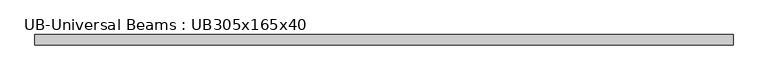
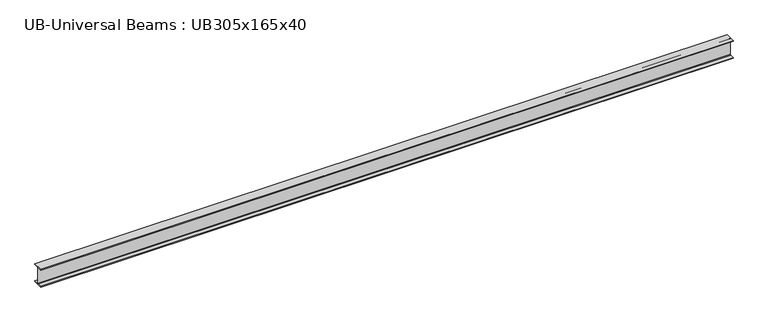
"""IFC4 building model written with IfcOpenShell, lengths in millimetres: member geometry, UB-Universal Beams : UB305x165x40."""

import ifcopenshell
import ifcopenshell.guid

model = None  # the IFC model being written
_history = None  # IfcOwnerHistory: only IFC2X3 demands one
_inside = {}  # id of a spatial element -> (the spatial element, [elements in it])
_under = {}  # id of a project, library or spatial element -> (it, [spatial elements below it])
_declared = {}  # id of a project -> (the project, [libraries it declares])
_typed = {}  # id of a type object -> (the type object, [elements of that type])
_made_of = {}  # id of a material, layer set ... -> (it, [elements and type objects made of it])


def new_model(schema):
    """Start an empty IFC model of exactly this schema.

    Asked for "IFC4X3", IfcOpenShell would pick the latest addendum, in which some entities
    have other attributes; the version numbers below select the first issue.
    IFC2X3 requires an IfcOwnerHistory on every rooted entity: one is made here for all.
    """
    global model, _history
    if schema == "IFC4X3":
        model = ifcopenshell.file(schema_version=(4, 3, 0, 0))
    else:
        model = ifcopenshell.file(schema=schema)
    _inside.clear()
    _under.clear()
    _declared.clear()
    _typed.clear()
    _made_of.clear()
    _history = None
    if model.schema == "IFC2X3":
        org = make("IfcOrganization", Name="unknown")
        user = make(
            "IfcPersonAndOrganization",
            ThePerson=make("IfcPerson", FamilyName="unknown"),
            TheOrganization=org,
        )
        app = make(
            "IfcApplication",
            ApplicationDeveloper=org,
            Version="unknown",
            ApplicationFullName="unknown",
            ApplicationIdentifier="unknown",
        )
        _history = make(
            "IfcOwnerHistory",
            OwningUser=user,
            OwningApplication=app,
            ChangeAction="ADDED",
            CreationDate=0,
        )
    return model


def make(cls, **values):
    """One entity of the class cls with the attributes given. An attribute that is None is left unset."""
    return model.create_entity(
        cls, **{name: value for name, value in values.items() if value is not None}
    )


def rooted(cls, **values):
    """An entity with a GlobalId (a new one), such as an element, a storey or a relation."""
    return make(cls, GlobalId=ifcopenshell.guid.new(), OwnerHistory=_history, **values)


def si_unit(unit_type, name, prefix=None):
    """IfcSIUnit, for example si_unit("LENGTHUNIT", "METRE", prefix="MILLI")."""
    return make("IfcSIUnit", UnitType=unit_type, Prefix=prefix, Name=name)


def assignment(units):
    """IfcUnitAssignment: the units of a project."""
    return None if units is None else make("IfcUnitAssignment", Units=units)


def point(xyz):
    """IfcCartesianPoint."""
    return None if xyz is None else make("IfcCartesianPoint", Coordinates=xyz)


def direction(xyz):
    """IfcDirection."""
    return None if xyz is None else make("IfcDirection", DirectionRatios=xyz)


def frame(location, z_axis=None, x_axis=None):
    """IfcAxis2Placement3D, a coordinate frame: its origin and axes. An axis left out is left unset."""
    return make(
        "IfcAxis2Placement3D",
        Location=point(location),
        Axis=direction(z_axis),
        RefDirection=direction(x_axis),
    )


def frame_2d(location, x_axis=None):
    """IfcAxis2Placement2D, a coordinate frame in the plane: its origin and x axis."""
    return make(
        "IfcAxis2Placement2D", Location=point(location), RefDirection=direction(x_axis)
    )


def origin():
    """The frame at (0, 0, 0) with its axes left unset."""
    return frame((0.0, 0.0, 0.0))


def place(relative_to, where):
    """IfcLocalPlacement: puts the frame where relative to a parent placement (None: the world)."""
    return make(
        "IfcLocalPlacement", PlacementRelTo=relative_to, RelativePlacement=where
    )


def context(
    kind, dimensions, precision=None, world=None, true_north=None, identifier=None
):
    """IfcGeometricRepresentationContext, for example the 3D "Model" context."""
    return make(
        "IfcGeometricRepresentationContext",
        ContextIdentifier=identifier,
        ContextType=kind,
        CoordinateSpaceDimension=dimensions,
        Precision=precision,
        WorldCoordinateSystem=world,
        TrueNorth=true_north,
    )


def project(units=None, contexts=None):
    """IfcProject with its units and contexts."""
    return rooted(
        "IfcProject",
        Name="project",
        RepresentationContexts=contexts,
        UnitsInContext=assignment(units),
    )


def spatial(cls, under=None, at=None, **own):
    """A site, building, storey or space (cls), placed at a placement, below another one or the project."""
    s = rooted(cls, ObjectPlacement=at, **own)
    if under is not None:
        _under.setdefault(under.id(), (under, []))[1].append(s)
    return s


def polyline(points):
    """IfcPolyline through the points."""
    return make("IfcPolyline", Points=[point(p) for p in points])


def circle_curve(where, radius):
    """IfcCircle in the frame where."""
    return make("IfcCircle", Position=where, Radius=radius)


def trimmed(basis, trim1, trim2, sense, master):
    """IfcTrimmedCurve: the piece of a basis curve between two trims."""
    return make(
        "IfcTrimmedCurve",
        BasisCurve=basis,
        Trim1=trim1,
        Trim2=trim2,
        SenseAgreement=sense,
        MasterRepresentation=master,
    )


def segment(curve, same_sense, transition):
    """IfcCompositeCurveSegment."""
    return make(
        "IfcCompositeCurveSegment",
        Transition=transition,
        SameSense=same_sense,
        ParentCurve=curve,
    )


def composite_curve(segments, self_intersect=None):
    """IfcCompositeCurve: segments joined end to end."""
    return make("IfcCompositeCurve", Segments=segments, SelfIntersect=self_intersect)


def outline(outer, holes=None, kind="AREA"):
    """IfcArbitraryClosedProfileDef: a profile drawn as a closed curve; with holes, ...WithVoids."""
    if holes is None:
        return make("IfcArbitraryClosedProfileDef", ProfileType=kind, OuterCurve=outer)
    return make(
        "IfcArbitraryProfileDefWithVoids",
        ProfileType=kind,
        OuterCurve=outer,
        InnerCurves=holes,
    )


def extrude(swept, where, along, depth):
    """IfcExtrudedAreaSolid: the profile swept, set in the frame where, extruded along a direction by depth."""
    return make(
        "IfcExtrudedAreaSolid",
        SweptArea=swept,
        Position=where,
        ExtrudedDirection=direction(along),
        Depth=depth,
    )


def shape(context_of_items, identifier, shape_type, items):
    """IfcShapeRepresentation: the items that make up one representation, for example the "Body"."""
    return make(
        "IfcShapeRepresentation",
        ContextOfItems=context_of_items,
        RepresentationIdentifier=identifier,
        RepresentationType=shape_type,
        Items=items,
    )


def source(mapping_origin, context_of_items, identifier, shape_type, items):
    """IfcRepresentationMap: a shape defined once, which mapped items show again and again."""
    return make(
        "IfcRepresentationMap",
        MappingOrigin=mapping_origin,
        MappedRepresentation=shape(context_of_items, identifier, shape_type, items),
    )


def transform(
    local_origin,
    x_axis=None,
    y_axis=None,
    z_axis=None,
    scale=None,
    scale2=None,
    scale3=None,
    uniform=True,
):
    """IfcCartesianTransformationOperator3D, or its non-uniform kind. x_axis, y_axis, z_axis: its Axis1, 2, 3."""
    if uniform:
        return make(
            "IfcCartesianTransformationOperator3D",
            Axis1=direction(x_axis),
            Axis2=direction(y_axis),
            LocalOrigin=point(local_origin),
            Scale=scale,
            Axis3=direction(z_axis),
        )
    return make(
        "IfcCartesianTransformationOperator3DnonUniform",
        Axis1=direction(x_axis),
        Axis2=direction(y_axis),
        LocalOrigin=point(local_origin),
        Scale=scale,
        Axis3=direction(z_axis),
        Scale2=scale2,
        Scale3=scale3,
    )


def mapped(mapping_source, mapping_target):
    """IfcMappedItem: shows the shape of a source again, moved by a transform."""
    return make(
        "IfcMappedItem", MappingSource=mapping_source, MappingTarget=mapping_target
    )


def made_of(thing, what):
    """Note that an element or type object is made of a material, layer set ...; save() writes the relation."""
    if what is not None:
        _made_of.setdefault(what.id(), (what, []))[1].append(thing)
    return thing


def element(
    cls,
    number,
    at=None,
    inside=None,
    cuts=None,
    type_object=None,
    material=None,
    context=None,
    identifier="Body",
    shape_type=None,
    held_by="IfcProductDefinitionShape",
    body=None,
    shapes=None,
    **own,
):
    """One element of the class cls, such as IfcWall. Its Tag is "e" and its number.

    at: its placement. inside: the storey or other place that contains it. cuts: it is an
    opening in that element (IfcRelVoidsElement). A single representation is given by context,
    identifier, shape_type and body (its items); several are given by shapes. held_by: the class
    of the entity that holds the representations. save() writes the other relations.
    """
    e = rooted(cls, Tag="e%d" % number, ObjectPlacement=at, **own)
    if body is not None:
        shapes = [shape(context, identifier, shape_type, body)]
    if shapes is not None:
        e.Representation = make(held_by, Representations=shapes)
    if inside is not None:
        _inside.setdefault(inside.id(), (inside, []))[1].append(e)
    if cuts is not None:
        rooted(
            "IfcRelVoidsElement", RelatingBuildingElement=cuts, RelatedOpeningElement=e
        )
    if type_object is not None:
        _typed.setdefault(type_object.id(), (type_object, []))[1].append(e)
    return made_of(e, material)


def aggregate(whole, parts):
    """IfcRelAggregates: a whole, such as a stair, and the parts it consists of."""
    return rooted("IfcRelAggregates", RelatingObject=whole, RelatedObjects=parts)


def save(model, path):
    """Write the relations noted so far, then the file.

    IfcRelAggregates (storeys below a building ...), IfcRelContainedInSpatialStructure (elements
    in a storey), IfcRelDefinesByType, IfcRelAssociatesMaterial and IfcRelDeclares: one each for
    every whole, place, type object, material and project.
    """
    for whole, parts in _under.values():
        aggregate(whole, parts)
    for where, things in _inside.values():
        rooted(
            "IfcRelContainedInSpatialStructure",
            RelatedElements=things,
            RelatingStructure=where,
        )
    for kind, things in _typed.values():
        rooted("IfcRelDefinesByType", RelatedObjects=things, RelatingType=kind)
    for what, things in _made_of.values():
        rooted("IfcRelAssociatesMaterial", RelatedObjects=things, RelatingMaterial=what)
    for by, libraries in _declared.values():
        rooted("IfcRelDeclares", RelatingContext=by, RelatedDefinitions=libraries)
    model.write(path)


def ub_universal_beams_ub305x165x40_967f8f3f(model_context):
    return source(origin(), model_context, "Body", "SweptSolid", [
        extrude(outline(composite_curve([segment(polyline([(82.5, -141.5), (82.5, -151.7), (-82.5, -151.7), (-82.5, -141.5), (-11.9, -141.5)]), True, "CONTINUOUS"), segment(trimmed(circle_curve(frame_2d((-11.9, -132.6)), 8.9), [point((-11.9, -141.5))], [point((-3.0, -132.6))], True, "CARTESIAN"), True, "CONTINUOUS"), segment(polyline([(-3.0, -132.6), (-3.0, 132.6)]), True, "CONTINUOUS"), segment(trimmed(circle_curve(frame_2d((-11.9, 132.6)), 8.9), [point((-3.0, 132.6))], [point((-11.9, 141.5))], True, "CARTESIAN"), True, "CONTINUOUS"), segment(polyline([(-11.9, 141.5), (-82.5, 141.5), (-82.5, 151.7), (82.5, 151.7), (82.5, 141.5), (11.9, 141.5)]), True, "CONTINUOUS"), segment(trimmed(circle_curve(frame_2d((11.9, 132.6)), 8.9), [point((11.9, 141.5))], [point((3.0, 132.6))], True, "CARTESIAN"), True, "CONTINUOUS"), segment(polyline([(3.0, 132.6), (3.0, -132.6)]), True, "CONTINUOUS"), segment(trimmed(circle_curve(frame_2d((11.9, -132.6)), 8.9), [point((3.0, -132.6))], [point((11.9, -141.5))], True, "CARTESIAN"), True, "CONTINUOUS"), segment(polyline([(11.9, -141.5), (82.5, -141.5)]), True, "CONTINUOUS")], self_intersect=False)), frame((-5621.7, 0.0, 0.0), z_axis=(1.0, 0.0, 0.0), x_axis=(0.0, 1.0, 0.0)), (0.0, 0.0, 1.0), 11304.3),
    ])


if __name__ == "__main__":
    model = new_model("IFC4")
    model_context = context("Model", 3, world=origin())
    ifc_project = project(units=[si_unit("LENGTHUNIT", "METRE", prefix="MILLI")], contexts=[model_context])
    site = spatial("IfcSite", under=ifc_project)
    building = spatial("IfcBuilding", under=site)
    placement = place(None, origin())
    ub_universal_beams_ub305x165x40_shape = ub_universal_beams_ub305x165x40_967f8f3f(model_context)
    element("IfcMember", 1, ObjectType="UB-Universal Beams : UB305x165x40", at=placement, inside=building, context=model_context, shape_type="MappedRepresentation", body=[
        mapped(ub_universal_beams_ub305x165x40_shape, transform((0.0, 0.0, 0.0), x_axis=(1.0, 0.0, 0.0), y_axis=(0.0, 1.0, 0.0), z_axis=(0.0, 0.0, 1.0))),
    ])
    save(model, "model.ifc")

# Revit data of these elements
# Type "UB-Universal Beams : UB305x165x40"
#   Section Name Key = "UB305X165X40"
#   Width = 16.5 cm
#   Web Thickness = 0.6 cm
#   Web Fillet = 0.89 cm
#   Warping Constant = 164000.0 cm⁶
#   Torsional Moment of Inertia = 14.70 cm⁴
#   Section Area = 51.3 cm²
#   Plastic Modulus weak axis = 142.0 cm³
#   Plastic Modulus strong axis = 623.0 cm³
#   Nominal Weight = 40.2999 kgf/m
#   Moment of Inertia weak axis = 764.00 cm⁴
#   Moment of Inertia strong axis = 8503.00 cm⁴
#   Height = 30.34 cm
#   Flange Thickness = 1.02 cm
#   Elastic Modulus weak axis = 92.6 cm³
#   Elastic Modulus strong axis = 560.0 cm³
#   Centroid Vertical = 15.17 cm
#   Centroid Horizontal = 8.25 cm
#   Bolt Spacing = 9.0 cm
#   Length [instance default] = 1500 mm
#   Structural Material [instance default] = Metal - Steel 43-275
#   Type Comments = ""
#   Assembly Code = ""
# Element 1 (IfcMember, "UB-Universal Beams : UB305x165x40")
#   Materials on its faces: "Metal - Steel 43-275"
# Materials
#   "Metal - Steel 43-275": class "Metal", colour RGB 247 247 247, transparency 0, Cost = 0
